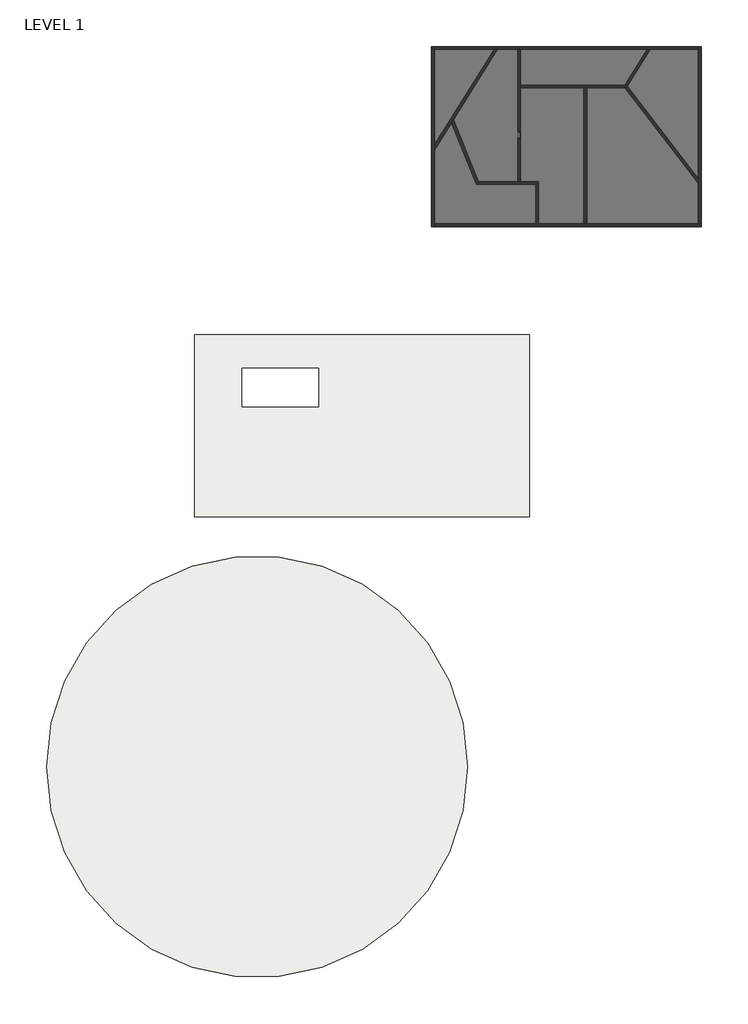
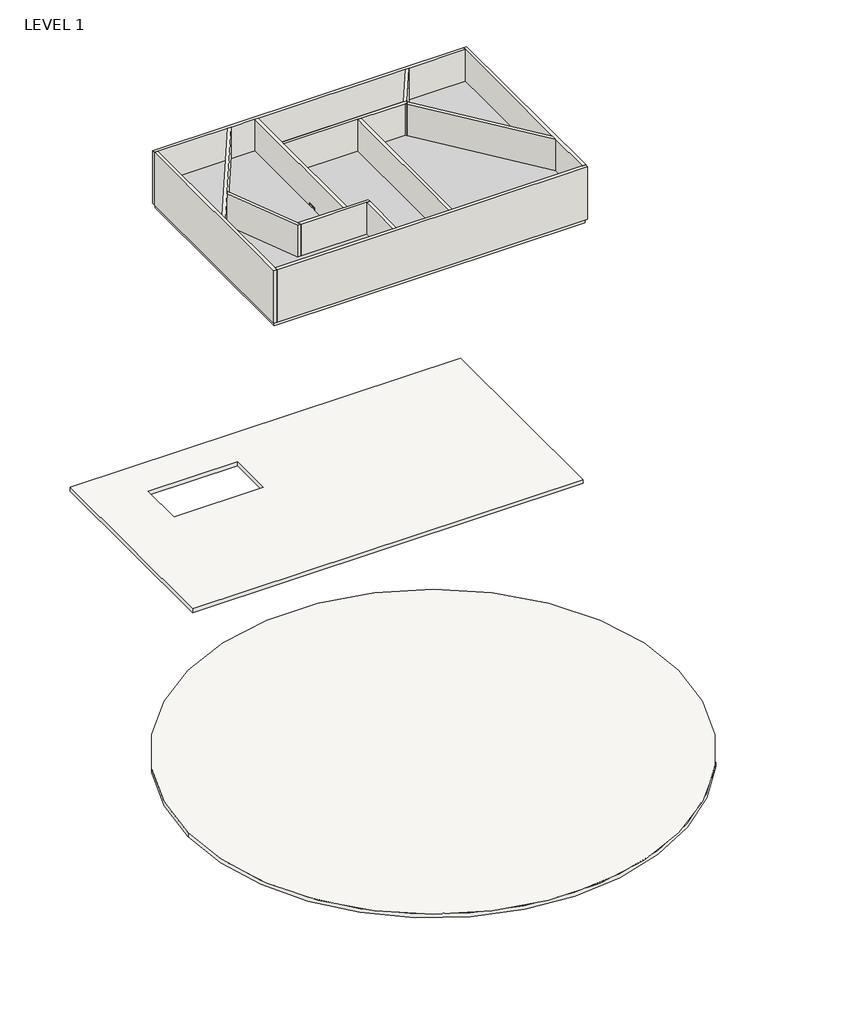
# One storey: 13 walls, 7 proxies, 3 slabs, 1 door.
"""IFC4 building model written with IfcOpenShell, lengths in millimetres."""

import ifcopenshell
import ifcopenshell.guid

model = None  # the IFC model being written
_history = None  # IfcOwnerHistory: only IFC2X3 demands one
_inside = {}  # id of a spatial element -> (the spatial element, [elements in it])
_under = {}  # id of a project, library or spatial element -> (it, [spatial elements below it])
_declared = {}  # id of a project -> (the project, [libraries it declares])
_typed = {}  # id of a type object -> (the type object, [elements of that type])
_made_of = {}  # id of a material, layer set ... -> (it, [elements and type objects made of it])


def new_model(schema):
    """Start an empty IFC model of exactly this schema.

    Asked for "IFC4X3", IfcOpenShell would pick the latest addendum, in which some entities
    have other attributes; the version numbers below select the first issue.
    IFC2X3 requires an IfcOwnerHistory on every rooted entity: one is made here for all.
    """
    global model, _history
    if schema == "IFC4X3":
        model = ifcopenshell.file(schema_version=(4, 3, 0, 0))
    else:
        model = ifcopenshell.file(schema=schema)
    _inside.clear()
    _under.clear()
    _declared.clear()
    _typed.clear()
    _made_of.clear()
    _history = None
    if model.schema == "IFC2X3":
        org = make("IfcOrganization", Name="unknown")
        user = make(
            "IfcPersonAndOrganization",
            ThePerson=make("IfcPerson", FamilyName="unknown"),
            TheOrganization=org,
        )
        app = make(
            "IfcApplication",
            ApplicationDeveloper=org,
            Version="unknown",
            ApplicationFullName="unknown",
            ApplicationIdentifier="unknown",
        )
        _history = make(
            "IfcOwnerHistory",
            OwningUser=user,
            OwningApplication=app,
            ChangeAction="ADDED",
            CreationDate=0,
        )
    return model


def make(cls, **values):
    """One entity of the class cls with the attributes given. An attribute that is None is left unset."""
    return model.create_entity(
        cls, **{name: value for name, value in values.items() if value is not None}
    )


def rooted(cls, **values):
    """An entity with a GlobalId (a new one), such as an element, a storey or a relation."""
    return make(cls, GlobalId=ifcopenshell.guid.new(), OwnerHistory=_history, **values)


def si_unit(unit_type, name, prefix=None):
    """IfcSIUnit, for example si_unit("LENGTHUNIT", "METRE", prefix="MILLI")."""
    return make("IfcSIUnit", UnitType=unit_type, Prefix=prefix, Name=name)


def assignment(units):
    """IfcUnitAssignment: the units of a project."""
    return None if units is None else make("IfcUnitAssignment", Units=units)


def point(xyz):
    """IfcCartesianPoint."""
    return None if xyz is None else make("IfcCartesianPoint", Coordinates=xyz)


def direction(xyz):
    """IfcDirection."""
    return None if xyz is None else make("IfcDirection", DirectionRatios=xyz)


def frame(location, z_axis=None, x_axis=None):
    """IfcAxis2Placement3D, a coordinate frame: its origin and axes. An axis left out is left unset."""
    return make(
        "IfcAxis2Placement3D",
        Location=point(location),
        Axis=direction(z_axis),
        RefDirection=direction(x_axis),
    )


def frame_2d(location, x_axis=None):
    """IfcAxis2Placement2D, a coordinate frame in the plane: its origin and x axis."""
    return make(
        "IfcAxis2Placement2D", Location=point(location), RefDirection=direction(x_axis)
    )


def origin():
    """The frame at (0, 0, 0) with its axes left unset."""
    return frame((0.0, 0.0, 0.0))


def origin_with_axes():
    """The frame at (0, 0, 0) with the z axis (0, 0, 1) and the x axis (1, 0, 0) written out."""
    return frame((0.0, 0.0, 0.0), z_axis=(0.0, 0.0, 1.0), x_axis=(1.0, 0.0, 0.0))


def place(relative_to, where):
    """IfcLocalPlacement: puts the frame where relative to a parent placement (None: the world)."""
    return make(
        "IfcLocalPlacement", PlacementRelTo=relative_to, RelativePlacement=where
    )


def context(
    kind, dimensions, precision=None, world=None, true_north=None, identifier=None
):
    """IfcGeometricRepresentationContext, for example the 3D "Model" context."""
    return make(
        "IfcGeometricRepresentationContext",
        ContextIdentifier=identifier,
        ContextType=kind,
        CoordinateSpaceDimension=dimensions,
        Precision=precision,
        WorldCoordinateSystem=world,
        TrueNorth=true_north,
    )


def project(units=None, contexts=None):
    """IfcProject with its units and contexts."""
    return rooted(
        "IfcProject",
        Name="project",
        RepresentationContexts=contexts,
        UnitsInContext=assignment(units),
    )


def spatial(cls, under=None, at=None, **own):
    """A site, building, storey or space (cls), placed at a placement, below another one or the project."""
    s = rooted(cls, ObjectPlacement=at, **own)
    if under is not None:
        _under.setdefault(under.id(), (under, []))[1].append(s)
    return s


def polyline(points):
    """IfcPolyline through the points."""
    return make("IfcPolyline", Points=[point(p) for p in points])


def circle_curve(where, radius):
    """IfcCircle in the frame where."""
    return make("IfcCircle", Position=where, Radius=radius)


def ellipse_curve(where, semi_axis1, semi_axis2):
    """IfcEllipse in the frame where."""
    return make(
        "IfcEllipse", Position=where, SemiAxis1=semi_axis1, SemiAxis2=semi_axis2
    )


def trimmed(basis, trim1, trim2, sense, master):
    """IfcTrimmedCurve: the piece of a basis curve between two trims."""
    return make(
        "IfcTrimmedCurve",
        BasisCurve=basis,
        Trim1=trim1,
        Trim2=trim2,
        SenseAgreement=sense,
        MasterRepresentation=master,
    )


def segment(curve, same_sense, transition):
    """IfcCompositeCurveSegment."""
    return make(
        "IfcCompositeCurveSegment",
        Transition=transition,
        SameSense=same_sense,
        ParentCurve=curve,
    )


def composite_curve(segments, self_intersect=None):
    """IfcCompositeCurve: segments joined end to end."""
    return make("IfcCompositeCurve", Segments=segments, SelfIntersect=self_intersect)


def outline(outer, holes=None, kind="AREA"):
    """IfcArbitraryClosedProfileDef: a profile drawn as a closed curve; with holes, ...WithVoids."""
    if holes is None:
        return make("IfcArbitraryClosedProfileDef", ProfileType=kind, OuterCurve=outer)
    return make(
        "IfcArbitraryProfileDefWithVoids",
        ProfileType=kind,
        OuterCurve=outer,
        InnerCurves=holes,
    )


def extrude(swept, where, along, depth):
    """IfcExtrudedAreaSolid: the profile swept, set in the frame where, extruded along a direction by depth."""
    return make(
        "IfcExtrudedAreaSolid",
        SweptArea=swept,
        Position=where,
        ExtrudedDirection=direction(along),
        Depth=depth,
    )


def faces_of(points, faces, orient=None, outer=None):
    """IfcFace entities. A face is a list of loops; a loop is a list of indices into points, from 0.

    orient and outer hold one flag for each loop. By default every Orientation is true, the
    first loop of a face is its IfcFaceOuterBound and the others are IfcFaceBound.
    """
    made = []
    for i, loops in enumerate(faces):
        bounds = []
        for j, loop in enumerate(loops):
            is_outer = j == 0 if outer is None else outer[i][j]
            bounds.append(
                make(
                    "IfcFaceOuterBound" if is_outer else "IfcFaceBound",
                    Bound=make("IfcPolyLoop", Polygon=[points[k] for k in loop]),
                    Orientation=True if orient is None else orient[i][j],
                )
            )
        made.append(make("IfcFace", Bounds=bounds))
    return made


def faceted_brep(points, faces, orient=None, outer=None, voids=None):
    """IfcFacetedBrep: a solid bounded by flat faces; with voids (closed shells), ...WithVoids."""
    shared = [point(p) for p in points]
    hull = make("IfcClosedShell", CfsFaces=faces_of(shared, faces, orient, outer))
    if voids is None:
        return make("IfcFacetedBrep", Outer=hull)
    return make(
        "IfcFacetedBrepWithVoids",
        Outer=hull,
        Voids=[
            make(cls, CfsFaces=faces_of(shared, fs, o, b)) for cls, fs, o, b in voids
        ],
    )


def shape(context_of_items, identifier, shape_type, items):
    """IfcShapeRepresentation: the items that make up one representation, for example the "Body"."""
    return make(
        "IfcShapeRepresentation",
        ContextOfItems=context_of_items,
        RepresentationIdentifier=identifier,
        RepresentationType=shape_type,
        Items=items,
    )


def source(mapping_origin, context_of_items, identifier, shape_type, items):
    """IfcRepresentationMap: a shape defined once, which mapped items show again and again."""
    return make(
        "IfcRepresentationMap",
        MappingOrigin=mapping_origin,
        MappedRepresentation=shape(context_of_items, identifier, shape_type, items),
    )


def transform(
    local_origin,
    x_axis=None,
    y_axis=None,
    z_axis=None,
    scale=None,
    scale2=None,
    scale3=None,
    uniform=True,
):
    """IfcCartesianTransformationOperator3D, or its non-uniform kind. x_axis, y_axis, z_axis: its Axis1, 2, 3."""
    if uniform:
        return make(
            "IfcCartesianTransformationOperator3D",
            Axis1=direction(x_axis),
            Axis2=direction(y_axis),
            LocalOrigin=point(local_origin),
            Scale=scale,
            Axis3=direction(z_axis),
        )
    return make(
        "IfcCartesianTransformationOperator3DnonUniform",
        Axis1=direction(x_axis),
        Axis2=direction(y_axis),
        LocalOrigin=point(local_origin),
        Scale=scale,
        Axis3=direction(z_axis),
        Scale2=scale2,
        Scale3=scale3,
    )


def mapped(mapping_source, mapping_target):
    """IfcMappedItem: shows the shape of a source again, moved by a transform."""
    return make(
        "IfcMappedItem", MappingSource=mapping_source, MappingTarget=mapping_target
    )


def made_of(thing, what):
    """Note that an element or type object is made of a material, layer set ...; save() writes the relation."""
    if what is not None:
        _made_of.setdefault(what.id(), (what, []))[1].append(thing)
    return thing


def element(
    cls,
    number,
    at=None,
    inside=None,
    cuts=None,
    type_object=None,
    material=None,
    context=None,
    identifier="Body",
    shape_type=None,
    held_by="IfcProductDefinitionShape",
    body=None,
    shapes=None,
    **own,
):
    """One element of the class cls, such as IfcWall. Its Tag is "e" and its number.

    at: its placement. inside: the storey or other place that contains it. cuts: it is an
    opening in that element (IfcRelVoidsElement). A single representation is given by context,
    identifier, shape_type and body (its items); several are given by shapes. held_by: the class
    of the entity that holds the representations. save() writes the other relations.
    """
    e = rooted(cls, Tag="e%d" % number, ObjectPlacement=at, **own)
    if body is not None:
        shapes = [shape(context, identifier, shape_type, body)]
    if shapes is not None:
        e.Representation = make(held_by, Representations=shapes)
    if inside is not None:
        _inside.setdefault(inside.id(), (inside, []))[1].append(e)
    if cuts is not None:
        rooted(
            "IfcRelVoidsElement", RelatingBuildingElement=cuts, RelatedOpeningElement=e
        )
    if type_object is not None:
        _typed.setdefault(type_object.id(), (type_object, []))[1].append(e)
    return made_of(e, material)


def aggregate(whole, parts):
    """IfcRelAggregates: a whole, such as a stair, and the parts it consists of."""
    return rooted("IfcRelAggregates", RelatingObject=whole, RelatedObjects=parts)


def save(model, path):
    """Write the relations noted so far, then the file.

    IfcRelAggregates (storeys below a building ...), IfcRelContainedInSpatialStructure (elements
    in a storey), IfcRelDefinesByType, IfcRelAssociatesMaterial and IfcRelDeclares: one each for
    every whole, place, type object, material and project.
    """
    for whole, parts in _under.values():
        aggregate(whole, parts)
    for where, things in _inside.values():
        rooted(
            "IfcRelContainedInSpatialStructure",
            RelatedElements=things,
            RelatingStructure=where,
        )
    for kind, things in _typed.values():
        rooted("IfcRelDefinesByType", RelatedObjects=things, RelatingType=kind)
    for what, things in _made_of.values():
        rooted("IfcRelAssociatesMaterial", RelatedObjects=things, RelatingMaterial=what)
    for by, libraries in _declared.values():
        rooted("IfcRelDeclares", RelatingContext=by, RelatedDefinitions=libraries)
    model.write(path)


def plane_surface(at):
    """IfcPlane: the flat surface through the origin of the frame at, square to its z axis."""
    return make("IfcPlane", Position=at)


def cylinder_surface(at, radius):
    """IfcCylindricalSurface: all points at the distance radius from the z axis of the frame at."""
    return make("IfcCylindricalSurface", Position=at, Radius=radius)


def advanced_brep(points, edges, surfaces, faces):
    """IfcAdvancedBrep: a solid bounded by faces that lie on surfaces and meet in shared edges.

    An edge is (start, end): straight between two places in points (the first is 0);
    or (start, end, curve); or (start, end, curve, False) where it runs against its curve.
    A face is (place in surfaces, loops), or (place, loops, False) where it looks against
    its surface's normal. A loop lists edges by number (the first is 1), with a minus sign
    where the edge is run from its end to its start. The first loop is the outer one.
    """
    corners = [point(p) for p in points]
    vertices = [make("IfcVertexPoint", VertexGeometry=c) for c in corners]
    made = []
    for start, end, *more in edges:
        made.append(
            make(
                "IfcEdgeCurve",
                EdgeStart=vertices[start],
                EdgeEnd=vertices[end],
                EdgeGeometry=more[0] if more else make("IfcPolyline", Points=[corners[start], corners[end]]),
                SameSense=more[1] if len(more) > 1 else True,
            )
        )
    hull = []
    for where, loops, *sense in faces:
        bounds = []
        for j, loop in enumerate(loops):
            ring = [make("IfcOrientedEdge", EdgeElement=made[abs(k) - 1], Orientation=k > 0) for k in loop]
            bounds.append(
                make(
                    "IfcFaceOuterBound" if j == 0 else "IfcFaceBound",
                    Bound=make("IfcEdgeLoop", EdgeList=ring),
                    Orientation=True,
                )
            )
        hull.append(make("IfcAdvancedFace", Bounds=bounds, FaceSurface=surfaces[where], SameSense=sense[0] if sense else True))
    return make("IfcAdvancedBrep", Outer=make("IfcClosedShell", CfsFaces=hull))


def generic_36_x_106_78535582(model_context):
    return source(origin(), model_context, "Body", "SolidModel", [
        advanced_brep(
        [(-393.7, 182.5625, 965.2), (-368.3, 182.5625, 965.2), (-368.3, 233.3625, 965.2), (-393.7, 258.7625, 965.2), (-254.0, 233.3625, 965.2), (-228.6, 258.7625, 965.2), (-228.6, 201.6125, 965.2), (-254.0, 201.6125, 965.2)],
        [
            (0, 1, circle_curve(frame((-381.0, 182.5625, 965.2), z_axis=(0.0, -1.0, 0.0), x_axis=(1.0, 0.0, 0.0)), 12.7)),
            (1, 0, circle_curve(frame((-381.0, 182.5625, 965.2), z_axis=(0.0, -1.0, 0.0), x_axis=(1.0, 0.0, 0.0)), 12.7)),
            (1, 2),
            (2, 3, ellipse_curve(frame((-381.0, 246.0625, 965.2), z_axis=(-0.7071067811867366, -0.7071067811863584, 0.0), x_axis=(0.7071067811863585, -0.7071067811867366, 0.0)), 17.9605122, 12.7)),
            (3, 0),
            (3, 2, ellipse_curve(frame((-381.0, 246.0625, 965.2), z_axis=(-0.7071067811867366, -0.7071067811863584, 0.0), x_axis=(0.7071067811863585, -0.7071067811867366, 0.0)), 17.9605122, 12.7)),
            (2, 4),
            (4, 5, ellipse_curve(frame((-241.3, 246.0625, 965.2), z_axis=(-0.7071067811863584, 0.7071067811867366, 0.0), x_axis=(-0.7071067811867366, -0.7071067811863585, 0.0)), 17.9605122, 12.7)),
            (5, 3),
            (5, 4, ellipse_curve(frame((-241.3, 246.0625, 965.2), z_axis=(-0.7071067811863584, 0.7071067811867366, 0.0), x_axis=(-0.7071067811867366, -0.7071067811863585, 0.0)), 17.9605122, 12.7)),
            (6, 7, circle_curve(frame((-241.3, 201.6125, 965.2), z_axis=(0.0, -1.0, 0.0), x_axis=(-1.0, 0.0, 0.0)), 12.7)),
            (7, 6, circle_curve(frame((-241.3, 201.6125, 965.2), z_axis=(0.0, -1.0, 0.0), x_axis=(-1.0, 0.0, 0.0)), 12.7)),
            (4, 7),
            (6, 5),
        ],
        [
            plane_surface(frame((-381.0, 182.5625, 965.2), z_axis=(0.0, -1.0, 0.0), x_axis=(0.0, 0.0, 1.0))),
            cylinder_surface(frame((-381.0, 182.5625, 965.2), z_axis=(0.0, -1.0, 0.0), x_axis=(1.0, 0.0, 0.0)), 12.7),
            cylinder_surface(frame((-381.0, 246.0625, 965.2), z_axis=(-1.0, 0.0, 0.0), x_axis=(0.0, -1.0, 0.0)), 12.7),
            plane_surface(frame((-241.3, 201.6125, 965.2), z_axis=(0.0, -1.0, 0.0), x_axis=(0.0, 0.0, 1.0))),
            cylinder_surface(frame((-241.3, 246.0625, 965.2), z_axis=(0.0, 1.0, 0.0), x_axis=(-1.0, 0.0, 0.0)), 12.7),
        ],
        [
            (0, [[1, 2]]),
            (1, [[3, 4, 5, -2]]),
            (1, [[-5, 6, -3, -1]]),
            (2, [[7, 8, 9, -4]]),
            (2, [[-9, 10, -7, -6]]),
            (3, [[11, 12]]),
            (4, [[13, -11, 14, -8]]),
            (4, [[-14, -12, -13, -10]]),
        ],
    ),
        extrude(outline(composite_curve([segment(trimmed(circle_curve(frame_2d((965.2, -381.0)), 25.4), [point((965.2, -406.4))], [point((965.2, -355.6))], False, "CARTESIAN"), True, "CONTINUOUS"), segment(trimmed(circle_curve(frame_2d((965.2, -381.0)), 25.4), [point((965.2, -355.6))], [point((965.2, -406.4))], False, "CARTESIAN"), True, "CONTINUOUS")], self_intersect=False)), frame((0.0, 176.2125, 0.0), z_axis=(0.0, 1.0, 0.0), x_axis=(0.0, 0.0, 1.0)), (0.0, 0.0, 1.0), 6.35),
        advanced_brep(
        [(-393.7, 125.4125, 965.2), (-368.3, 125.4125, 965.2), (-393.7, 49.2125, 965.2), (-368.3, 74.6125, 965.2), (-228.6, 49.2125, 965.2), (-254.0, 74.6125, 965.2), (-228.6, 106.3625, 965.2), (-254.0, 106.3625, 965.2)],
        [
            (0, 1, circle_curve(frame((-381.0, 125.4125, 965.2), z_axis=(0.0, 1.0, 0.0), x_axis=(1.0, 0.0, 0.0)), 12.7)),
            (1, 0, circle_curve(frame((-381.0, 125.4125, 965.2), z_axis=(0.0, 1.0, 0.0), x_axis=(1.0, 0.0, 0.0)), 12.7)),
            (0, 2),
            (2, 3, ellipse_curve(frame((-381.0, 61.9125, 965.2), z_axis=(-0.7071067811867366, 0.7071067811863584, 0.0), x_axis=(0.7071067811863585, 0.7071067811867366, 0.0)), 17.9605122, 12.7)),
            (3, 1),
            (3, 2, ellipse_curve(frame((-381.0, 61.9125, 965.2), z_axis=(-0.7071067811867366, 0.7071067811863584, 0.0), x_axis=(0.7071067811863585, 0.7071067811867366, 0.0)), 17.9605122, 12.7)),
            (2, 4),
            (4, 5, ellipse_curve(frame((-241.3, 61.9125, 965.2), z_axis=(-0.7071067811863584, -0.7071067811867366, 0.0), x_axis=(-0.7071067811867366, 0.7071067811863585, 0.0)), 17.9605122, 12.7)),
            (5, 3),
            (5, 4, ellipse_curve(frame((-241.3, 61.9125, 965.2), z_axis=(-0.7071067811863584, -0.7071067811867366, 0.0), x_axis=(-0.7071067811867366, 0.7071067811863585, 0.0)), 17.9605122, 12.7)),
            (6, 7, circle_curve(frame((-241.3, 106.3625, 965.2), z_axis=(0.0, 1.0, 0.0), x_axis=(-1.0, 0.0, 0.0)), 12.7)),
            (7, 6, circle_curve(frame((-241.3, 106.3625, 965.2), z_axis=(0.0, 1.0, 0.0), x_axis=(-1.0, 0.0, 0.0)), 12.7)),
            (4, 6),
            (7, 5),
        ],
        [
            plane_surface(frame((-381.0, 125.4125, 965.2), z_axis=(0.0, 1.0, 0.0), x_axis=(0.0, 0.0, 1.0))),
            cylinder_surface(frame((-381.0, 125.4125, 965.2), z_axis=(0.0, 1.0, 0.0), x_axis=(1.0, 0.0, 0.0)), 12.7),
            cylinder_surface(frame((-381.0, 61.9125, 965.2), z_axis=(-1.0, 0.0, 0.0), x_axis=(0.0, 1.0, 0.0)), 12.7),
            plane_surface(frame((-241.3, 106.3625, 965.2), z_axis=(0.0, 1.0, 0.0), x_axis=(0.0, 0.0, 1.0))),
            cylinder_surface(frame((-241.3, 61.9125, 965.2), z_axis=(0.0, -1.0, 0.0), x_axis=(-1.0, 0.0, 0.0)), 12.7),
        ],
        [
            (0, [[1, 2]]),
            (1, [[-1, 3, 4, 5]]),
            (1, [[-2, -5, 6, -3]]),
            (2, [[-4, 7, 8, 9]]),
            (2, [[-6, -9, 10, -7]]),
            (3, [[11, 12]]),
            (4, [[-8, 13, -12, 14]]),
            (4, [[-10, -14, -11, -13]]),
        ],
    ),
        extrude(outline(composite_curve([segment(trimmed(circle_curve(frame_2d((965.2, -381.0)), 25.4), [point((965.2, -406.4))], [point((965.2, -355.6))], False, "CARTESIAN"), True, "CONTINUOUS"), segment(trimmed(circle_curve(frame_2d((965.2, -381.0)), 25.4), [point((965.2, -355.6))], [point((965.2, -406.4))], False, "CARTESIAN"), True, "CONTINUOUS")], self_intersect=False)), frame((0.0, 125.4125, 0.0), z_axis=(0.0, 1.0, 0.0), x_axis=(0.0, 0.0, 1.0)), (0.0, 0.0, 1.0), 6.35),
        extrude(outline(polyline([(127.0, 150.8125), (-127.0, 150.8125), (-127.0, 157.1625), (127.0, 157.1625), (127.0, 150.8125)])), frame((0.0, 0.0, 1549.4), z_axis=(0.0, 0.0, 1.0), x_axis=(1.0, 0.0, 0.0)), (0.0, 0.0, 1.0), 254.0),
        extrude(outline(polyline([(1828.8, 152.4), (1828.8, -152.4), (1524.0, -152.4), (1524.0, 152.4), (1828.8, 152.4)]), holes=[polyline([(1803.4, 127.0), (1549.4, 127.0), (1549.4, -127.0), (1803.4, -127.0), (1803.4, 127.0)])]), frame((0.0, 131.7625, 0.0), z_axis=(0.0, 1.0, 0.0), x_axis=(0.0, 0.0, 1.0)), (0.0, 0.0, 1.0), 44.45),
        extrude(outline(polyline([(2692.4, -457.2), (0.0, -457.2), (0.0, 457.2), (2692.4, 457.2), (2692.4, -457.2)]), holes=[polyline([(1828.8, 152.4), (1524.0, 152.4), (1524.0, -152.4), (1828.8, -152.4), (1828.8, 152.4)])]), frame((0.0, 131.7625, 0.0), z_axis=(0.0, 1.0, 0.0), x_axis=(0.0, 0.0, 1.0)), (0.0, 0.0, 1.0), 44.45),
        extrude(outline(polyline([(2743.2, 508.0), (2743.2, -508.0), (0.0, -508.0), (0.0, -457.2), (2692.4, -457.2), (2692.4, 457.2), (0.0, 457.2), (0.0, 508.0), (2743.2, 508.0)])), frame((0.0, -176.2125, 0.0), z_axis=(0.0, 1.0, 0.0), x_axis=(0.0, 0.0, 1.0)), (0.0, 0.0, 1.0), 352.425),
    ])


model = new_model("IFC4")

# Units and contexts
model_context = context("Model", 3, world=origin())
ifc_project = project(units=[si_unit("LENGTHUNIT", "METRE", prefix="MILLI")], contexts=[model_context])

# Site, building, storey
site = spatial("IfcSite", under=ifc_project)
building = spatial("IfcBuilding", under=site)
storey = spatial("IfcBuildingStorey", under=building, Name="LEVEL 1", Elevation=0.0)

# Proxies
placement = place(None, origin())
element("IfcBuildingElementProxy", 1, Name="297845 : Bath 1", ObjectType="297845 : Bath 1", at=placement, inside=storey, context=model_context, shape_type="SweptSolid", body=[
    extrude(outline(polyline([(-15983.6198287, 1891.5541178), (-18047.5905904, -1411.4895592), (-18047.5905904, 10762.1019471), (-10440.6863555, 10762.1019471), (-15983.6198287, 1891.5541178)])), origin_with_axes(), (0.0, 0.0, 1.0), 2438.4),
])
element("IfcBuildingElementProxy", 2, Name="297848 : Room 1", ObjectType="297848 : Room 1", at=placement, inside=storey, context=model_context, shape_type="SweptSolid", body=[
    extrude(outline(polyline([(-15983.6198287, 1891.5541178), (-18047.5905904, -1411.4895592), (-18047.5905904, 10762.1019471), (-10440.6863555, 10762.1019471), (-15983.6198287, 1891.5541178)])), origin_with_axes(), (0.0, 0.0, 1.0), 2438.4),
    extrude(outline(polyline([(-7446.0755979, 6037.7019471), (-7446.0755979, -6079.8724884), (-12461.1937659, -6079.8724884), (-15637.167808, 1780.9391101), (-10025.1144067, 10762.1019471), (-7446.0755979, 10762.1019471), (-7446.0755979, 6037.7019471)])), origin_with_axes(), (0.0, 0.0, 1.0), 2438.4),
])
element("IfcBuildingElementProxy", 3, Name="297851 : Room 3", ObjectType="297851 : Room 3", at=placement, inside=storey, context=model_context, shape_type="SweptSolid", body=[
    extrude(outline(polyline([(-15868.011904, 1411.5113325), (-12698.9074299, -6432.2974884), (-7269.8630979, -6432.2974884), (-5136.2630979, -6432.2974884), (-5136.2630979, -11440.6730529), (-18047.5905904, -11440.6730529), (-18047.5905904, -2076.5436981), (-15868.011904, 1411.5113325)])), origin_with_axes(), (0.0, 0.0, 1.0), 2438.4),
])
element("IfcBuildingElementProxy", 4, Name="297854 : Living 4", ObjectType="297854 : Living 4", at=placement, inside=storey, context=model_context, shape_type="SweptSolid", body=[
    extrude(outline(polyline([(-4783.8380979, -6079.8724884), (-7093.6505979, -6079.8724884), (-7093.6505979, 5861.4894471), (983.5494021, 5861.4894471), (983.5494021, -11440.6730529), (-4783.8380979, -11440.6730529), (-4783.8380979, -6079.8724884)])), origin_with_axes(), (0.0, 0.0, 1.0), 2438.4),
])
element("IfcBuildingElementProxy", 5, Name="297857 : Office 5", ObjectType="297857 : Office 5", at=placement, inside=storey, context=model_context, shape_type="SweptSolid", body=[
    extrude(outline(polyline([(6196.0607184, 6213.9144471), (1159.7619021, 6213.9144471), (-7093.6505979, 6213.9144471), (-7093.6505979, 10762.1019471), (9038.0836939, 10762.1019471), (6196.0607184, 6213.9144471)])), origin_with_axes(), (0.0, 0.0, 1.0), 2438.4),
])
element("IfcBuildingElementProxy", 6, Name="297860 : Office 6", ObjectType="297860 : Office 6", at=placement, inside=storey, context=model_context, shape_type="SweptSolid", body=[
    extrude(outline(polyline([(1335.9744021, 5861.4894471), (6207.0305501, 5861.4894471), (15585.1844096, -6316.0734677), (15585.1844096, -11440.6730529), (1335.9744021, -11440.6730529), (1335.9744021, 5861.4894471)])), origin_with_axes(), (0.0, 0.0, 1.0), 2438.4),
])
element("IfcBuildingElementProxy", 7, Name="297863 : Room 7", ObjectType="297863 : Room 7", at=placement, inside=storey, context=model_context, shape_type="SweptSolid", body=[
    extrude(outline(polyline([(15585.1844096, -5738.4715145), (6508.0738542, 6048.1857029), (9453.6556427, 10762.1019471), (15585.1844096, 10762.1019471), (15585.1844096, -5738.4715145)])), origin_with_axes(), (0.0, 0.0, 1.0), 2438.4),
])

# Door
generic_36_x_106_shape = generic_36_x_106_78535582(model_context)
element("IfcDoor", 8, ObjectType="V_SingleFlush_HOK_I : Generic 36 x 106", at=placement, inside=storey, context=model_context, shape_type="MappedRepresentation", body=[
    mapped(generic_36_x_106_shape, transform((-7269.8630979, -109.1915207, 0.0), x_axis=(0.0, -1.0, 0.0), y_axis=(1.0, 0.0, 0.0), z_axis=(0.0, 0.0, 1.0))),
])

# Slabs
element("IfcSlab", 9, ObjectType="Steel Bar Joist 14\" - VCT on Concrete", at=placement, inside=storey, context=model_context, shape_type="SweptSolid", body=[
    extrude(outline(polyline([(15761.3969096, 10938.3144471), (15761.3969096, -11616.8855529), (-18223.8030904, -11616.8855529), (-18223.8030904, 10938.3144471), (15761.3969096, 10938.3144471)])), frame((0.0, 0.0, -441.325), z_axis=(0.0, 0.0, 1.0), x_axis=(1.0, 0.0, 0.0)), (0.0, 0.0, 1.0), 441.325),
])
element("IfcSlab", 10, ObjectType="Steel Bar Joist 14\" - VCT on Concrete", at=placement, inside=storey, context=model_context, shape_type="SweptSolid", body=[
    extrude(outline(polyline([(-5930.6831108, -25585.0154861), (-5930.6831108, -48749.8154861), (-48602.6831108, -48749.8154861), (-48602.6831108, -25585.0154861), (-5930.6831108, -25585.0154861)]), holes=[polyline([(-32790.0042795, -29843.5813483), (-42543.6042795, -29843.5813483), (-42543.6042795, -34720.3813483), (-32790.0042795, -34720.3813483), (-32790.0042795, -29843.5813483)])]), frame((0.0, 0.0, -441.325), z_axis=(0.0, 0.0, 1.0), x_axis=(1.0, 0.0, 0.0)), (0.0, 0.0, 1.0), 441.325),
])
element("IfcSlab", 11, ObjectType="Steel Bar Joist 14\" - VCT on Concrete", at=placement, inside=storey, context=model_context, shape_type="SweptSolid", body=[
    extrude(outline(composite_curve([segment(trimmed(circle_curve(frame_2d((-40643.129322, -80564.4235698)), 26822.4), [point((-67465.529322, -80564.4235698))], [point((-13820.729322, -80564.4235698))], False, "CARTESIAN"), True, "CONTINUOUS"), segment(trimmed(circle_curve(frame_2d((-40643.129322, -80564.4235698)), 26822.4), [point((-13820.729322, -80564.4235698))], [point((-67465.529322, -80564.4235698))], False, "CARTESIAN"), True, "CONTINUOUS")], self_intersect=False)), frame((0.0, 0.0, -441.325), z_axis=(0.0, 0.0, 1.0), x_axis=(1.0, 0.0, 0.0)), (0.0, 0.0, 1.0), 441.325),
])

# Walls
element("IfcWall", 12, ObjectType="_Exterior - Brick on Mtl. Stud", at=placement, inside=storey, context=model_context, shape_type="Brep", body=[
    faceted_brep([(-18400.0155904, 10762.1019471, 0.0), (-18047.5905904, 10762.1019471, 0.0), (-10440.6863555, 10762.1019471, 0.0), (-10025.1144067, 10762.1019471, 0.0), (-7446.0755979, 10762.1019471, 0.0), (-7093.6505979, 10762.1019471, 0.0), (9038.0836939, 10762.1019471, 0.0), (9453.6556427, 10762.1019471, 0.0), (15585.1844096, 10762.1019471, 0.0), (15585.1844096, 10762.1019471, 6096.0), (9453.6556427, 10762.1019471, 6096.0), (9038.0836939, 10762.1019471, 6096.0), (-7093.6505979, 10762.1019471, 6096.0), (-7446.0755979, 10762.1019471, 6096.0), (-10025.1144067, 10762.1019471, 6096.0), (-10440.6863555, 10762.1019471, 6096.0), (-18047.5905904, 10762.1019471, 6096.0), (-18400.0155904, 10762.1019471, 6096.0), (-18400.0155904, 11114.5269471, 0.0), (-18400.0155904, 11114.5269471, 6096.0), (15585.1844096, 11114.5269471, 6096.0), (15585.1844096, 11114.5269471, 0.0)], [[[0, 1, 2, 3, 4, 5, 6, 7, 8, 9, 10, 11, 12, 13, 14, 15, 16, 17]], [[18, 19, 20, 21]], [[8, 7, 6, 5, 4, 3, 2, 1, 0, 18, 21]], [[17, 16, 15, 14, 13, 12, 11, 10, 9, 20, 19]], [[0, 17, 19, 18]], [[9, 8, 21, 20]]]),
])
element("IfcWall", 13, ObjectType="_Exterior - Brick on Mtl. Stud", at=placement, inside=storey, context=model_context, shape_type="Brep", body=[
    faceted_brep([(-18047.5905904, -11793.0980529, 0.0), (-18047.5905904, -11440.6730529, 0.0), (-18047.5905904, -2076.5436981, 0.0), (-18047.5905904, -1411.4895592, 0.0), (-18047.5905904, 10762.1019471, 0.0), (-18047.5905904, 10762.1019471, 6096.0), (-18047.5905904, -1411.4895592, 6096.0), (-18047.5905904, -2076.5436981, 6096.0), (-18047.5905904, -11440.6730529, 6096.0), (-18047.5905904, -11793.0980529, 6096.0), (-18400.0155904, -11793.0980529, 0.0), (-18400.0155904, -11793.0980529, 6096.0), (-18400.0155904, 10762.1019471, 6096.0), (-18400.0155904, 10762.1019471, 0.0)], [[[0, 1, 2, 3, 4, 5, 6, 7, 8, 9]], [[10, 11, 12, 13]], [[4, 3, 2, 1, 0, 10, 13]], [[9, 8, 7, 6, 5, 12, 11]], [[0, 9, 11, 10]], [[5, 4, 13, 12]]]),
])
element("IfcWall", 14, ObjectType="_Exterior - Brick on Mtl. Stud", at=placement, inside=storey, context=model_context, shape_type="Brep", body=[
    faceted_brep([(15937.6094096, -11440.6730529, 0.0), (15585.1844096, -11440.6730529, 0.0), (1335.9744021, -11440.6730529, 0.0), (983.5494021, -11440.6730529, 0.0), (-4783.8380979, -11440.6730529, 0.0), (-5136.2630979, -11440.6730529, 0.0), (-18047.5905904, -11440.6730529, 0.0), (-18047.5905904, -11440.6730529, 6096.0), (-5136.2630979, -11440.6730529, 6096.0), (-4783.8380979, -11440.6730529, 6096.0), (983.5494021, -11440.6730529, 6096.0), (1335.9744021, -11440.6730529, 6096.0), (15585.1844096, -11440.6730529, 6096.0), (15937.6094096, -11440.6730529, 6096.0), (15937.6094096, -11793.0980529, 0.0), (15937.6094096, -11793.0980529, 6096.0), (-18047.5905904, -11793.0980529, 6096.0), (-18047.5905904, -11793.0980529, 0.0)], [[[0, 1, 2, 3, 4, 5, 6, 7, 8, 9, 10, 11, 12, 13]], [[14, 15, 16, 17]], [[6, 5, 4, 3, 2, 1, 0, 14, 17]], [[13, 12, 11, 10, 9, 8, 7, 16, 15]], [[0, 13, 15, 14]], [[7, 6, 17, 16]]]),
])
element("IfcWall", 15, ObjectType="_Exterior - Brick on Mtl. Stud", at=placement, inside=storey, context=model_context, shape_type="Brep", body=[
    faceted_brep([(15585.1844096, 11114.5269471, 0.0), (15585.1844096, 10762.1019471, 0.0), (15585.1844096, -5738.4715145, 0.0), (15585.1844096, -6316.0734677, 0.0), (15585.1844096, -11440.6730529, 0.0), (15585.1844096, -11440.6730529, 6096.0), (15585.1844096, -6316.0734677, 6096.0), (15585.1844096, -5738.4715145, 6096.0), (15585.1844096, 10762.1019471, 6096.0), (15585.1844096, 11114.5269471, 6096.0), (15937.6094096, 11114.5269471, 0.0), (15937.6094096, 11114.5269471, 6096.0), (15937.6094096, -11440.6730529, 6096.0), (15937.6094096, -11440.6730529, 0.0)], [[[0, 1, 2, 3, 4, 5, 6, 7, 8, 9]], [[10, 11, 12, 13]], [[4, 3, 2, 1, 0, 10, 13]], [[9, 8, 7, 6, 5, 12, 11]], [[0, 9, 11, 10]], [[5, 4, 13, 12]]]),
])
element("IfcWall", 16, ObjectType="_Exterior - Brick on Mtl. Stud", at=placement, inside=storey, context=model_context, shape_type="Brep", body=[
    faceted_brep([(-10440.6863555, 10762.1019471, 0.0), (-18047.5905904, -1411.4895592, 0.0), (-18047.5905904, -1411.4895592, 6096.0), (-10440.6863555, 10762.1019471, 6096.0), (-10025.1144067, 10762.1019471, 0.0), (-10025.1144067, 10762.1019471, 6096.0), (-15637.167808, 1780.9391101, 6096.0), (-15868.011904, 1411.5113325, 6096.0), (-18047.5905904, -2076.5436981, 6096.0), (-18047.5905904, -2076.5436981, 0.0), (-15868.011904, 1411.5113325, 0.0), (-15637.167808, 1780.9391101, 0.0)], [[[0, 1, 2, 3]], [[4, 5, 6, 7, 8, 9, 10, 11]], [[1, 0, 4, 11, 10, 9]], [[3, 2, 8, 7, 6, 5]], [[0, 3, 5, 4]], [[2, 1, 9, 8]]]),
])
element("IfcWall", 17, ObjectType="_Exterior - Brick on Mtl. Stud", at=placement, inside=storey, context=model_context, shape_type="Brep", body=[
    faceted_brep([(-15868.011904, 1411.5113325, 0.0), (-12698.9074299, -6432.2974884, 0.0), (-12698.9074299, -6432.2974884, 6096.0), (-15868.011904, 1411.5113325, 6096.0), (-15637.167808, 1780.9391101, 0.0), (-15637.167808, 1780.9391101, 6096.0), (-12461.1937659, -6079.8724884, 6096.0), (-12318.8048232, -6432.2974884, 6096.0), (-12318.8048232, -6432.2974884, 0.0), (-12461.1937659, -6079.8724884, 0.0)], [[[0, 1, 2, 3]], [[4, 5, 6, 7, 8, 9]], [[1, 0, 4, 9, 8]], [[3, 2, 7, 6, 5]], [[0, 3, 5, 4]], [[2, 1, 8, 7]]]),
])
element("IfcWall", 18, ObjectType="_Exterior - Brick on Mtl. Stud", at=placement, inside=storey, context=model_context, shape_type="Brep", body=[
    faceted_brep([(-12318.8048232, -6432.2974884, 0.0), (-5136.2630979, -6432.2974884, 0.0), (-4783.8380979, -6432.2974884, 0.0), (-4783.8380979, -6432.2974884, 6096.0), (-5136.2630979, -6432.2974884, 6096.0), (-12318.8048232, -6432.2974884, 6096.0), (-12461.1937659, -6079.8724884, 0.0), (-12461.1937659, -6079.8724884, 6096.0), (-7446.0755979, -6079.8724884, 6096.0), (-7093.6505979, -6079.8724884, 6096.0), (-4783.8380979, -6079.8724884, 6096.0), (-4783.8380979, -6079.8724884, 0.0), (-7093.6505979, -6079.8724884, 0.0), (-7446.0755979, -6079.8724884, 0.0)], [[[0, 1, 2, 3, 4, 5]], [[6, 7, 8, 9, 10, 11, 12, 13]], [[2, 1, 0, 6, 13, 12, 11]], [[5, 4, 3, 10, 9, 8, 7]], [[0, 5, 7, 6]], [[3, 2, 11, 10]]]),
])
element("IfcWall", 19, ObjectType="_Exterior - Brick on Mtl. Stud", at=placement, inside=storey, context=model_context, shape_type="SweptSolid", body=[
    extrude(outline(polyline([(-5136.2630979, -11440.6730529), (-5136.2630979, -6432.2974884), (-4783.8380979, -6432.2974884), (-4783.8380979, -11440.6730529), (-5136.2630979, -11440.6730529)])), origin_with_axes(), (0.0, 0.0, 1.0), 6096.0),
])
element("IfcWall", 20, ObjectType="_Exterior - Brick on Mtl. Stud", at=placement, inside=storey, context=model_context, shape_type="Brep", body=[
    faceted_brep([(-7446.0755979, -6079.8724884, 6096.0), (-7446.0755979, 10762.1019471, 6096.0), (-7446.0755979, 10762.1019471, 0.0), (-7446.0755979, 398.8084793, 0.0), (-7446.0755979, 398.8084793, 2743.2), (-7446.0755979, -617.1915207, 2743.2), (-7446.0755979, -617.1915207, 0.0), (-7446.0755979, -6079.8724884, 0.0), (-7093.6505979, 10762.1019471, 6096.0), (-7093.6505979, 6213.9144471, 6096.0), (-7093.6505979, 5861.4894471, 6096.0), (-7093.6505979, -6079.8724884, 6096.0), (-7093.6505979, -6079.8724884, 0.0), (-7093.6505979, -617.1915207, 0.0), (-7093.6505979, -617.1915207, 2743.2), (-7093.6505979, 398.8084793, 2743.2), (-7093.6505979, 398.8084793, 0.0), (-7093.6505979, 5861.4894471, 0.0), (-7093.6505979, 6213.9144471, 0.0), (-7093.6505979, 10762.1019471, 0.0)], [[[0, 1, 2, 3, 4, 5, 6, 7]], [[8, 9, 10, 11, 12, 13, 14, 15, 16, 17, 18, 19]], [[2, 19, 18, 17, 16, 3]], [[12, 7, 6, 13]], [[1, 0, 11, 10, 9, 8]], [[2, 1, 8, 19]], [[0, 7, 12, 11]], [[5, 14, 13, 6]], [[14, 5, 4, 15]], [[15, 4, 3, 16]]]),
])
element("IfcWall", 21, ObjectType="_Exterior - Brick on Mtl. Stud", at=placement, inside=storey, context=model_context, shape_type="Brep", body=[
    faceted_brep([(-7093.6505979, 5861.4894471, 0.0), (983.5494021, 5861.4894471, 0.0), (1335.9744021, 5861.4894471, 0.0), (6207.0305501, 5861.4894471, 0.0), (6391.4130858, 5861.4894471, 0.0), (6391.4130858, 5861.4894471, 6096.0), (6207.0305501, 5861.4894471, 6096.0), (1335.9744021, 5861.4894471, 6096.0), (983.5494021, 5861.4894471, 6096.0), (-7093.6505979, 5861.4894471, 6096.0), (-7093.6505979, 6213.9144471, 0.0), (-7093.6505979, 6213.9144471, 6096.0), (6196.0607184, 6213.9144471, 6096.0), (6611.6326672, 6213.9144471, 6096.0), (6611.6326672, 6213.9144471, 0.0), (6196.0607184, 6213.9144471, 0.0), (6508.0738542, 6048.1857029, 0.0), (6508.0738542, 6048.1857029, 6096.0)], [[[0, 1, 2, 3, 4, 5, 6, 7, 8, 9]], [[10, 11, 12, 13, 14, 15]], [[4, 3, 2, 1, 0, 10, 15, 14, 16]], [[9, 8, 7, 6, 5, 17, 13, 12, 11]], [[0, 9, 11, 10]], [[5, 4, 16, 14, 13, 17]]]),
])
element("IfcWall", 22, ObjectType="_Exterior - Brick on Mtl. Stud", at=placement, inside=storey, context=model_context, shape_type="SweptSolid", body=[
    extrude(outline(polyline([(9453.6556427, 10762.1019471), (6611.6326672, 6213.9144471), (6196.0607184, 6213.9144471), (9038.0836939, 10762.1019471), (9453.6556427, 10762.1019471)])), origin_with_axes(), (0.0, 0.0, 1.0), 6096.0),
])
element("IfcWall", 23, ObjectType="_Exterior - Brick on Mtl. Stud", at=placement, inside=storey, context=model_context, shape_type="SweptSolid", body=[
    extrude(outline(polyline([(15585.1844096, -6316.0734677), (6207.0305501, 5861.4894471), (6391.4130858, 5861.4894471), (6508.0738542, 6048.1857029), (15585.1844096, -5738.4715145), (15585.1844096, -6316.0734677)])), origin_with_axes(), (0.0, 0.0, 1.0), 6096.0),
])
element("IfcWall", 24, ObjectType="_Exterior - Brick on Mtl. Stud", at=placement, inside=storey, context=model_context, shape_type="SweptSolid", body=[
    extrude(outline(polyline([(983.5494021, -11440.6730529), (983.5494021, 5861.4894471), (1335.9744021, 5861.4894471), (1335.9744021, -11440.6730529), (983.5494021, -11440.6730529)])), origin_with_axes(), (0.0, 0.0, 1.0), 6096.0),
])

save(model, "model.ifc")

# Revit data of these elements
# Type "297845 : Bath 1"
#   Height [instance default] = 8' - 0"
#   Default Elevation = 4' - 0"
# Type "297848 : Room 1"
#   Height [instance default] = 8' - 0"
#   Default Elevation = 4' - 0"
# Type "297851 : Room 3"
#   Height [instance default] = 8' - 0"
#   Default Elevation = 4' - 0"
# Type "297854 : Living 4"
#   Height [instance default] = 8' - 0"
#   Default Elevation = 4' - 0"
# Type "297857 : Office 5"
#   Height [instance default] = 8' - 0"
#   Default Elevation = 4' - 0"
# Type "297860 : Office 6"
#   Height [instance default] = 8' - 0"
#   Default Elevation = 4' - 0"
# Type "297863 : Room 7"
#   Height [instance default] = 8' - 0"
#   Default Elevation = 4' - 0"
# Type "V_SingleFlush_HOK_I : Generic 36 x 106"
#   Type Mark = "23"
#   URL_BPD = "http://www.knowledgenet.hok.com/v6/HOK.App.Knet.Web/BPDDetail.aspx?UUID=a7282016-f650-cf84-99e3-8cf7c5ef63ab&Mode=User&ObjectType=2"
#   Manufacturer = "BPD LIBRARY"
#   Equipment = ""
#   DoorTypeMark = ""
#   DoorTypeDescription = ""
#   DoorTagRemark [instance default] = ""
#   DoorPanelType = "V"
#   DoorPanelMaterial = ""
#   DoorPanelGlassType = "GL-02"
#   DoorOpeningIdentifier = ""
#   DoorFrameType = "01"
#   DoorFrameMaterial = ""
#   BIM_ID = ""
#   Assembly Code = "C1020"
#   DoorSwingArc = 90.00°
#   DoorRoughWidth = 3' - 4"
#   DoorRoughHeight = 9' - 0"
#   DoorPanelWidth1 = 3' - 0"
#   DoorPanelThickness = 0' - 1 3/4"
#   DoorPanelHeight = 8' - 10"
#   DoorGlazingWidth = 0' - 10"
#   DoorGlazingMountingHeight = 5' - 1"
#   DoorGlazingHeight = 0' - 10"
#   DoorGlazingFrameWidth = 0' - 1"
#   DoorFrameJambThickness = 0' - 2"
#   DoorFrameHeadThickness = 0' - 2"
#   DoorPanelMaskingRegionVisibility = yes
#   RenderDoorPanel = Door - Panel - Generic
#   RenderDoorGlass = Door - Glazing - Generic
#   RenderDoorFrame = Door - Frame - Generic
#   URL = ""
#   Type Comments = ""
#   Rough Width = 0
#   Rough Height = 0
#   Model = ""
#   Function = (empty or 0)
#   Height = 0
#   Wall Closure = (empty or 0)
#   Width = 0
#   Fire Rating = ""
#   Description = (empty or 0)
#   Cost = 0
# Type "Steel Bar Joist 14\" - VCT on Concrete"
#   Assembly Code = "B1010"
#   Thickness = 1' - 5 3/8"
#   Function = 0
#   Layers, outside or top first: 0' - 0 1/4" "VCT - Vinyl Composition Tile" (function 5); 0' - 3" "Concrete - Cast-in-Place Lightweight Concrete" (function 1); 0' - 0 1/8" "Metal - Deck" (function 1); 1' - 2" "Structure - Steel Bar Joist Layer" (function 1)
# Type "_Exterior - Brick on Mtl. Stud"
#   Assembly Code = "B2010158"
#   Width = 1' - 1 7/8"
#   Layers, outside or top first: 0' - 3 5/8" "Masonry - Brick" (function 4); 0' - 3" "Misc. Air Layers - Air Space" (function 3); 0' - 0" "Air Barrier - Air Infiltration Barrier" (function 100); 0' - 0 3/4" "Wood - Sheathing - Plywood" (function 2); 0' - 6" "Metal - Stud Layer" (function 1); 0' - 0" "Vapor / Moisture Barriers - Vapor Retarder" (function 100); 0' - 0 1/2" "Finishes - Interior - Gypsum Wall Board" (function 5)
# Element 1 (IfcBuildingElementProxy, "297845 : Bath 1")
#   Height = 8' - 0"
#   Phase Created = New Construction
#   Materials on its faces: "Mass Room - Mech."
# Element 2 (IfcBuildingElementProxy, "297848 : Room 1")
#   Comments = "Office"
#   Height = 8' - 0"
#   Phase Created = New Construction
#   Materials on its faces: "Mass Room - test", "Mass Room - test2"
# Element 3 (IfcBuildingElementProxy, "297851 : Room 3")
#   Comments = "Office"
#   Height = 8' - 0"
#   Phase Created = New Construction
#   Materials on its faces: "Mass Room - test1"
# Element 4 (IfcBuildingElementProxy, "297854 : Living 4")
#   Comments = "Living"
#   Height = 8' - 0"
#   Phase Created = New Construction
#   Materials on its faces: "Mass Room - Living"
# Element 5 (IfcBuildingElementProxy, "297857 : Office 5")
#   Comments = "Conference"
#   Height = 8' - 0"
#   Phase Created = New Construction
#   Materials on its faces: "Mass Room - Office"
# Element 6 (IfcBuildingElementProxy, "297860 : Office 6")
#   Comments = "Living"
#   Height = 8' - 0"
#   Phase Created = New Construction
#   Materials on its faces: "Mass Room - Office"
# Element 7 (IfcBuildingElementProxy, "297863 : Room 7")
#   Comments = "Office"
#   Height = 8' - 0"
#   Phase Created = New Construction
#   Materials on its faces: "Mass Room - Conference"
# Element 8 (IfcDoor, "V_SingleFlush_HOK_I : Generic 36 x 106")
#   DoorTagRemark = ""
#   Phase Created = New Construction
#   Materials on its faces: "Door - Hardware - Generic", "Door - Panel - Generic", "Door - Frame - Generic", "Door - Glazing - Generic"
# Elements 9, 10, 11 (IfcSlab, "Steel Bar Joist 14\" - VCT on Concrete")
#   Height Offset From Level = 0' - 0"
#   Phase Created = New Construction
#   Materials on its faces: "Structure - Steel Bar Joist Layer", "VCT - Vinyl Composition Tile"
# Elements 12, 13, 14, 15, 18 (IfcWall, "_Exterior - Brick on Mtl. Stud")
#   Top Offset = 0' - 0"
#   Base Offset = 0' - 0"
#   Unconnected Height = 20' - 0"
#   wall height = 20' - 0"
#   Phase Created = New Construction
#   Base Constraint = LEVEL 1
#   Materials on its faces: "Default Wall", "Masonry - Brick", "Finishes - Interior - Gypsum Wall Board"
# Elements 16, 17, 19, 20, 21, 22, 23, 24 (IfcWall, "_Exterior - Brick on Mtl. Stud")
#   Top Offset = 0' - 0"
#   Base Offset = 0' - 0"
#   Unconnected Height = 20' - 0"
#   wall height = 20' - 0"
#   Phase Created = New Construction
#   Base Constraint = LEVEL 1
#   Materials on its faces: "Default Wall", "Finishes - Interior - Gypsum Wall Board", "Masonry - Brick"
# Materials
#   "Door - Panel - Generic": class "Unassigned", colour RGB 196 146 67, transparency 0, Comments = "Rendering appearance not upgraded "
#   "Door - Glazing - Generic": class "Unassigned", colour RGB 0 128 192, transparency 0.75
#   "Door - Frame - Generic": class "Unassigned", colour RGB 164 185 197, transparency 0, Comments = "Rendering appearance not upgraded "
#   "VCT - Vinyl Composition Tile": class "Vinyl", colour RGB 179 160 124, transparency 0, Description = "Interior finish"
#   "Concrete - Cast-in-Place Lightweight Concrete": class "Concrete", colour RGB 127 127 127, transparency 0
#   "Metal - Deck": class "Metal", colour RGB 199 199 199, transparency 0
#   "Structure - Steel Bar Joist Layer": class "Metal", colour RGB 127 127 127, transparency 0
#   "Masonry - Brick": class "Brick", colour RGB 170 98 104, transparency 0, Cost = 0
#   "Misc. Air Layers - Air Space": class "Miscellaneous", colour RGB 255 255 255, transparency 0
#   "Air Barrier - Air Infiltration Barrier": class "Miscellaneous", colour RGB 127 127 127, transparency 0
#   "Wood - Sheathing - Plywood": class "Unassigned", colour RGB 212 179 113, transparency 0, Description = "Plywood"
#   "Metal - Stud Layer": class "Metal", colour RGB 199 199 199, transparency 0
#   "Vapor / Moisture Barriers - Vapor Retarder": class "Miscellaneous", colour RGB 127 127 127, transparency 0
#   "Finishes - Interior - Gypsum Wall Board": class "Finishes", colour RGB 127 127 127, transparency 0, Comments = "Rendering appearance not upgraded ", Description = "GWB", Cost = 0
#   "Mass Room - Mech.": class "Unassigned", colour RGB 38 106 193, transparency 0.5
#   "Mass Room - test": class "Unassigned", colour RGB 126 173 184, transparency 0.5
#   "Mass Room - test2": class "Unassigned", colour RGB 34 251 137, transparency 0.5
#   "Mass Room - test1": class "Unassigned", colour RGB 126 173 184, transparency 0.5
#   "Mass Room - Living": class "Unassigned", colour RGB 234 83 155, transparency 0.5
#   "Mass Room - Office": class "Unassigned", colour RGB 163 166 84, transparency 0.5
#   "Mass Room - Conference": class "Unassigned", colour RGB 83 183 35, transparency 0.5
#   "Door - Hardware - Generic": class "Unassigned", colour RGB 164 185 197, transparency 0, Comments = "Rendering appearance not upgraded "
#   "Default Wall": class "Unassigned", colour RGB 128 128 128, transparency 0, Comments = "Rendering appearance not upgraded "
# Room at (-15993.543, 7991.185) mm, phase "New Construction", upper level "LEVEL 1", upper offset 8' - 0", lower offset 0' - 0"
#   Comments = ""
#   Department = "Mech."
#   Number = "1"
#   Name = "Bath"
#   Oscar Code = "1100"
#   OscarTitle = "Exterior Wall"
# Room at (-10417.893, 1300.405) mm, phase "New Construction", upper level "LEVEL 1", upper offset 8' - 0", lower offset 0' - 0"
#   Comments = "test"
#   Department = "Living"
#   Number = "2"
#   Name = "Living"
#   Oscar Code = "1320"
#   OscarTitle = "Stall"
# Room at (-14774.343, -8576.46) mm, phase "New Construction", upper level "LEVEL 1", upper offset 8' - 0", lower offset 0' - 0"
#   Comments = "test1"
#   Department = "Corridor"
#   Number = "3"
#   Name = "Hall"
#   Oscar Code = "1200"
#   OscarTitle = "Excluded"
# Room at (-3089.896, -531.594) mm, phase "New Construction", upper level "LEVEL 1", upper offset 8' - 0", lower offset 0' - 0"
#   Comments = "test"
#   Department = "Living"
#   Number = "4"
#   Name = "Living"
# Room at (494.45, 8958.458) mm, phase "New Construction", upper level "LEVEL 1", upper offset 8' - 0", lower offset 0' - 0"
#   Comments = "test2"
#   Department = "Office"
#   Number = "5"
#   Name = "Office"
# Room at (6946.273, -4115.94) mm, phase "New Construction", upper level "LEVEL 1", upper offset 8' - 0", lower offset 0' - 0"
#   Comments = "test"
#   Department = "Office"
#   Number = "6"
#   Name = "Office"
# Room at (12123.662, 5521.969) mm, phase "New Construction", upper level "LEVEL 1", upper offset 8' - 0", lower offset 0' - 0"
#   Comments = "test1"
#   Department = "Conference"
#   Number = "7"
#   Name = "Room"
# Area, not placed, upper offset 0' - 0", lower offset 0' - 0"
#   Name = "Area"
# Area at (12721.053, -19329.499) mm, upper offset 8' - 0", lower offset 0' - 0"
#   Number = "1"
#   Name = "Area"
# Area at (13358.271, -26338.887) mm, upper offset 8' - 0", lower offset 0' - 0"
#   Number = "2"
#   Name = "Area"
# Area at (8499.49, -34941.318) mm, upper offset 8' - 0", lower offset 0' - 0"
#   Number = "3"
#   Name = "Area"
